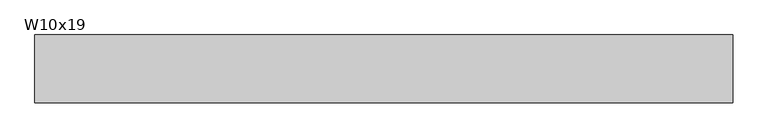
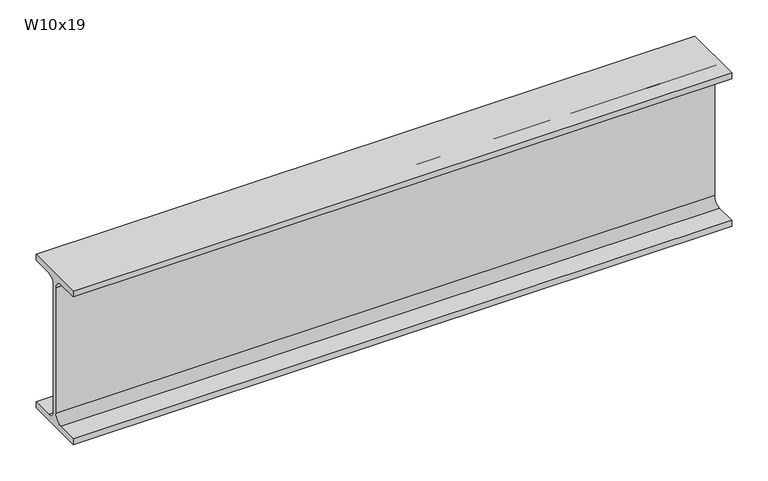
"""IFC4 building model written with IfcOpenShell, lengths in millimetres: beam geometry, RME W-Wide Flange : W10x19."""

from ifc_helpers import new_model, si_unit, point, frame, frame_2d, origin, place, context, project, spatial, polyline, circle_curve, trimmed, segment, composite_curve, outline, extrude, source, transform, mapped, element, save


def w10x19_ddde9493(model_context):
    return source(origin(), model_context, "Body", "SweptSolid", [
        extrude(outline(composite_curve([segment(polyline([(51.054, -119.507), (51.054, -129.54), (-51.054, -129.54), (-51.054, -119.507), (-16.9545, -119.507)]), True, "CONTINUOUS"), segment(trimmed(circle_curve(frame_2d((-16.9545, -105.7275)), 13.7795), [point((-16.9545, -119.507))], [point((-3.175, -105.7275))], True, "CARTESIAN"), True, "CONTINUOUS"), segment(polyline([(-3.175, -105.7275), (-3.175, 105.7275)]), True, "CONTINUOUS"), segment(trimmed(circle_curve(frame_2d((-16.9545, 105.7275)), 13.7795), [point((-3.175, 105.7275))], [point((-16.9545, 119.507))], True, "CARTESIAN"), True, "CONTINUOUS"), segment(polyline([(-16.9545, 119.507), (-51.054, 119.507), (-51.054, 129.54), (51.054, 129.54), (51.054, 119.507), (16.9545, 119.507)]), True, "CONTINUOUS"), segment(trimmed(circle_curve(frame_2d((16.9545, 105.7275)), 13.7795), [point((16.9545, 119.507))], [point((3.175, 105.7275))], True, "CARTESIAN"), True, "CONTINUOUS"), segment(polyline([(3.175, 105.7275), (3.175, -105.7275)]), True, "CONTINUOUS"), segment(trimmed(circle_curve(frame_2d((16.9545, -105.7275)), 13.7795), [point((3.175, -105.7275))], [point((16.9545, -119.507))], True, "CARTESIAN"), True, "CONTINUOUS"), segment(polyline([(16.9545, -119.507), (51.054, -119.507)]), True, "CONTINUOUS")], self_intersect=False)), frame((-519.2548697, 0.0, 0.0), z_axis=(1.0, 0.0, 0.0), x_axis=(0.0, 1.0, 0.0)), (0.0, 0.0, 1.0), 1051.20974),
    ])


if __name__ == "__main__":
    model = new_model("IFC4")
    model_context = context("Model", 3, world=origin())
    ifc_project = project(units=[si_unit("LENGTHUNIT", "METRE", prefix="MILLI")], contexts=[model_context])
    site = spatial("IfcSite", under=ifc_project)
    building = spatial("IfcBuilding", under=site)
    placement = place(None, origin())
    w10x19_shape = w10x19_ddde9493(model_context)
    element("IfcBeam", 1, ObjectType="RME W-Wide Flange : W10x19", at=placement, inside=building, context=model_context, shape_type="MappedRepresentation", body=[
        mapped(w10x19_shape, transform((0.0, 0.0, 0.0), x_axis=(1.0, 0.0, 0.0), y_axis=(0.0, 1.0, 0.0), z_axis=(0.0, 0.0, 1.0))),
    ])
    save(model, "model.ifc")

# Revit data of these elements
# Type "RME W-Wide Flange : W10x19"
#   WELD P [instance default] = ""
#   WELD LE [instance default] = ""
#   WELD D [instance default] = ""
#   TOP SECTION SIZE [instance default] = ""
#   TOP SECTION LENGTH [instance default] = ""
#   REMARKS [instance default] = ""
#   REINF TYPE [instance default] = ""
#   Nominal Size = "W24"
#   End Bearing Capacity [instance default] = ""
#   BOT SECTION SIZE [instance default] = ""
#   BOT SECTION LENGTH [instance default] = ""
#   Assembly Code = "B10"
#   W = 19
#   Start Extension Calculation [instance default] = 10' - 0"
#   Start Extension [instance default] = -0' - 0 1/2"
#   End Extension Calculation [instance default] = 10' - 0"
#   End Extension [instance default] = -0' - 0 1/2"
#   Length [instance default] = 5' - 0"
#   bf = 0' - 4.02"
#   d = 0' - 10.2"
#   k = 0' - 0 15/16"
#   k2 = 0' - 0.5425"
#   tf = 0' - 0.395"
#   tw = 0' - 0 1/4"
#   A = 0.0390278 SF
#   Structural Material [instance default] = Metal - Steel - ASTM A992
# Element 1 (IfcBeam, "RME W-Wide Flange : W10x19")
#   Materials on its faces: "Metal - Steel - ASTM A992"
# Materials
#   "Metal - Steel - ASTM A992": class "Metal", colour RGB 255 128 0, transparency 0
